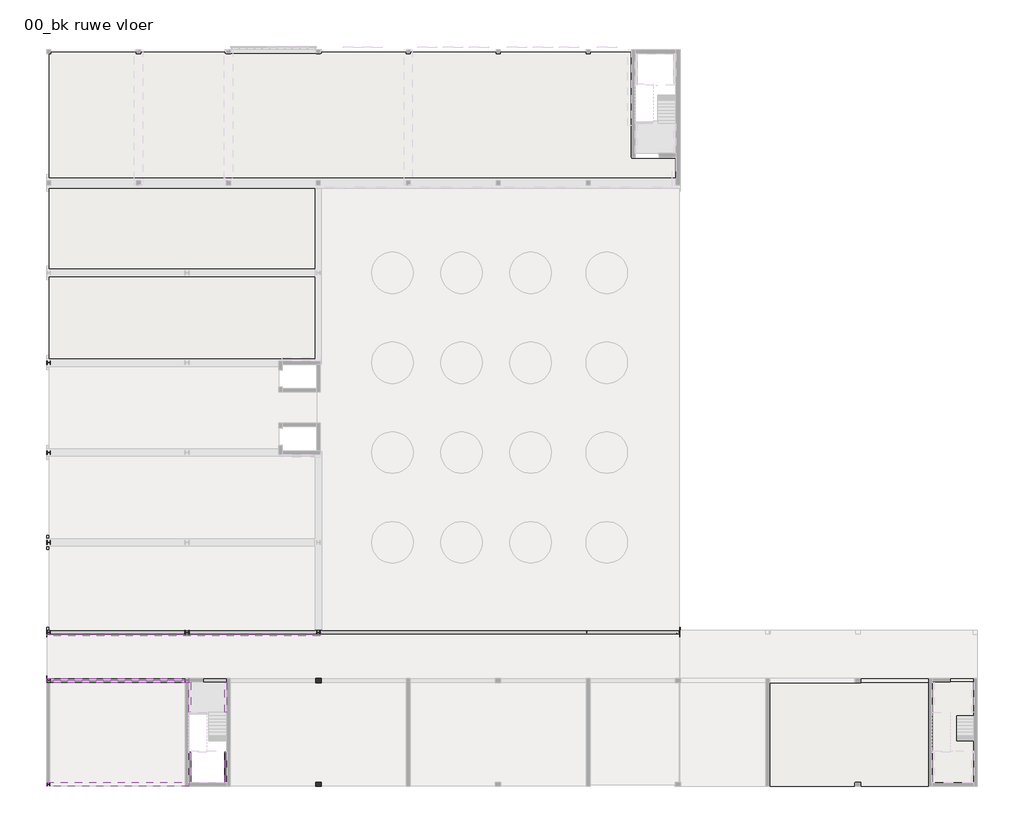
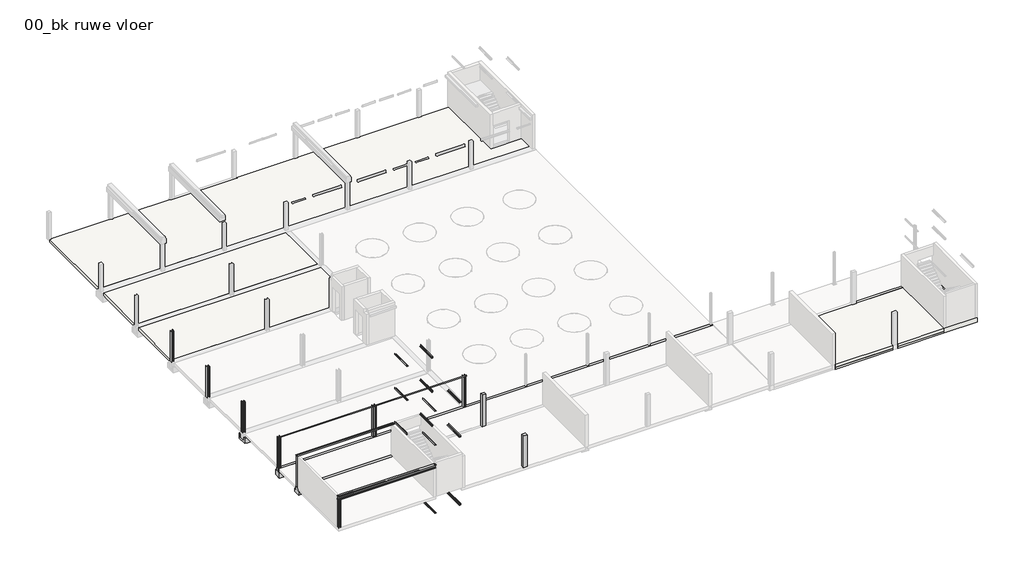
# One storey, part 4 of 6: 24 beams, 10 columns, 8 slabs.
"""IFC4 building model written with IfcOpenShell, lengths in millimetres."""

import ifcopenshell
import ifcopenshell.guid

model = None  # the IFC model being written
_history = None  # IfcOwnerHistory: only IFC2X3 demands one
_inside = {}  # id of a spatial element -> (the spatial element, [elements in it])
_under = {}  # id of a project, library or spatial element -> (it, [spatial elements below it])
_declared = {}  # id of a project -> (the project, [libraries it declares])
_typed = {}  # id of a type object -> (the type object, [elements of that type])
_made_of = {}  # id of a material, layer set ... -> (it, [elements and type objects made of it])


def new_model(schema):
    """Start an empty IFC model of exactly this schema.

    Asked for "IFC4X3", IfcOpenShell would pick the latest addendum, in which some entities
    have other attributes; the version numbers below select the first issue.
    IFC2X3 requires an IfcOwnerHistory on every rooted entity: one is made here for all.
    """
    global model, _history
    if schema == "IFC4X3":
        model = ifcopenshell.file(schema_version=(4, 3, 0, 0))
    else:
        model = ifcopenshell.file(schema=schema)
    _inside.clear()
    _under.clear()
    _declared.clear()
    _typed.clear()
    _made_of.clear()
    _history = None
    if model.schema == "IFC2X3":
        org = make("IfcOrganization", Name="unknown")
        user = make(
            "IfcPersonAndOrganization",
            ThePerson=make("IfcPerson", FamilyName="unknown"),
            TheOrganization=org,
        )
        app = make(
            "IfcApplication",
            ApplicationDeveloper=org,
            Version="unknown",
            ApplicationFullName="unknown",
            ApplicationIdentifier="unknown",
        )
        _history = make(
            "IfcOwnerHistory",
            OwningUser=user,
            OwningApplication=app,
            ChangeAction="ADDED",
            CreationDate=0,
        )
    return model


def make(cls, **values):
    """One entity of the class cls with the attributes given. An attribute that is None is left unset."""
    return model.create_entity(
        cls, **{name: value for name, value in values.items() if value is not None}
    )


def rooted(cls, **values):
    """An entity with a GlobalId (a new one), such as an element, a storey or a relation."""
    return make(cls, GlobalId=ifcopenshell.guid.new(), OwnerHistory=_history, **values)


def si_unit(unit_type, name, prefix=None):
    """IfcSIUnit, for example si_unit("LENGTHUNIT", "METRE", prefix="MILLI")."""
    return make("IfcSIUnit", UnitType=unit_type, Prefix=prefix, Name=name)


def assignment(units):
    """IfcUnitAssignment: the units of a project."""
    return None if units is None else make("IfcUnitAssignment", Units=units)


def point(xyz):
    """IfcCartesianPoint."""
    return None if xyz is None else make("IfcCartesianPoint", Coordinates=xyz)


def direction(xyz):
    """IfcDirection."""
    return None if xyz is None else make("IfcDirection", DirectionRatios=xyz)


def frame(location, z_axis=None, x_axis=None):
    """IfcAxis2Placement3D, a coordinate frame: its origin and axes. An axis left out is left unset."""
    return make(
        "IfcAxis2Placement3D",
        Location=point(location),
        Axis=direction(z_axis),
        RefDirection=direction(x_axis),
    )


def frame_2d(location, x_axis=None):
    """IfcAxis2Placement2D, a coordinate frame in the plane: its origin and x axis."""
    return make(
        "IfcAxis2Placement2D", Location=point(location), RefDirection=direction(x_axis)
    )


def origin():
    """The frame at (0, 0, 0) with its axes left unset."""
    return frame((0.0, 0.0, 0.0))


def place(relative_to, where):
    """IfcLocalPlacement: puts the frame where relative to a parent placement (None: the world)."""
    return make(
        "IfcLocalPlacement", PlacementRelTo=relative_to, RelativePlacement=where
    )


def context(
    kind, dimensions, precision=None, world=None, true_north=None, identifier=None
):
    """IfcGeometricRepresentationContext, for example the 3D "Model" context."""
    return make(
        "IfcGeometricRepresentationContext",
        ContextIdentifier=identifier,
        ContextType=kind,
        CoordinateSpaceDimension=dimensions,
        Precision=precision,
        WorldCoordinateSystem=world,
        TrueNorth=true_north,
    )


def project(units=None, contexts=None):
    """IfcProject with its units and contexts."""
    return rooted(
        "IfcProject",
        Name="project",
        RepresentationContexts=contexts,
        UnitsInContext=assignment(units),
    )


def spatial(cls, under=None, at=None, **own):
    """A site, building, storey or space (cls), placed at a placement, below another one or the project."""
    s = rooted(cls, ObjectPlacement=at, **own)
    if under is not None:
        _under.setdefault(under.id(), (under, []))[1].append(s)
    return s


def polyline(points):
    """IfcPolyline through the points."""
    return make("IfcPolyline", Points=[point(p) for p in points])


def circle_curve(where, radius):
    """IfcCircle in the frame where."""
    return make("IfcCircle", Position=where, Radius=radius)


def trimmed(basis, trim1, trim2, sense, master):
    """IfcTrimmedCurve: the piece of a basis curve between two trims."""
    return make(
        "IfcTrimmedCurve",
        BasisCurve=basis,
        Trim1=trim1,
        Trim2=trim2,
        SenseAgreement=sense,
        MasterRepresentation=master,
    )


def segment(curve, same_sense, transition):
    """IfcCompositeCurveSegment."""
    return make(
        "IfcCompositeCurveSegment",
        Transition=transition,
        SameSense=same_sense,
        ParentCurve=curve,
    )


def composite_curve(segments, self_intersect=None):
    """IfcCompositeCurve: segments joined end to end."""
    return make("IfcCompositeCurve", Segments=segments, SelfIntersect=self_intersect)


def outline(outer, holes=None, kind="AREA"):
    """IfcArbitraryClosedProfileDef: a profile drawn as a closed curve; with holes, ...WithVoids."""
    if holes is None:
        return make("IfcArbitraryClosedProfileDef", ProfileType=kind, OuterCurve=outer)
    return make(
        "IfcArbitraryProfileDefWithVoids",
        ProfileType=kind,
        OuterCurve=outer,
        InnerCurves=holes,
    )


def extrude(swept, where, along, depth):
    """IfcExtrudedAreaSolid: the profile swept, set in the frame where, extruded along a direction by depth."""
    return make(
        "IfcExtrudedAreaSolid",
        SweptArea=swept,
        Position=where,
        ExtrudedDirection=direction(along),
        Depth=depth,
    )


def faces_of(points, faces, orient=None, outer=None):
    """IfcFace entities. A face is a list of loops; a loop is a list of indices into points, from 0.

    orient and outer hold one flag for each loop. By default every Orientation is true, the
    first loop of a face is its IfcFaceOuterBound and the others are IfcFaceBound.
    """
    made = []
    for i, loops in enumerate(faces):
        bounds = []
        for j, loop in enumerate(loops):
            is_outer = j == 0 if outer is None else outer[i][j]
            bounds.append(
                make(
                    "IfcFaceOuterBound" if is_outer else "IfcFaceBound",
                    Bound=make("IfcPolyLoop", Polygon=[points[k] for k in loop]),
                    Orientation=True if orient is None else orient[i][j],
                )
            )
        made.append(make("IfcFace", Bounds=bounds))
    return made


def faceted_brep(points, faces, orient=None, outer=None, voids=None):
    """IfcFacetedBrep: a solid bounded by flat faces; with voids (closed shells), ...WithVoids."""
    shared = [point(p) for p in points]
    hull = make("IfcClosedShell", CfsFaces=faces_of(shared, faces, orient, outer))
    if voids is None:
        return make("IfcFacetedBrep", Outer=hull)
    return make(
        "IfcFacetedBrepWithVoids",
        Outer=hull,
        Voids=[
            make(cls, CfsFaces=faces_of(shared, fs, o, b)) for cls, fs, o, b in voids
        ],
    )


def shape(context_of_items, identifier, shape_type, items):
    """IfcShapeRepresentation: the items that make up one representation, for example the "Body"."""
    return make(
        "IfcShapeRepresentation",
        ContextOfItems=context_of_items,
        RepresentationIdentifier=identifier,
        RepresentationType=shape_type,
        Items=items,
    )


def source(mapping_origin, context_of_items, identifier, shape_type, items):
    """IfcRepresentationMap: a shape defined once, which mapped items show again and again."""
    return make(
        "IfcRepresentationMap",
        MappingOrigin=mapping_origin,
        MappedRepresentation=shape(context_of_items, identifier, shape_type, items),
    )


def transform(
    local_origin,
    x_axis=None,
    y_axis=None,
    z_axis=None,
    scale=None,
    scale2=None,
    scale3=None,
    uniform=True,
):
    """IfcCartesianTransformationOperator3D, or its non-uniform kind. x_axis, y_axis, z_axis: its Axis1, 2, 3."""
    if uniform:
        return make(
            "IfcCartesianTransformationOperator3D",
            Axis1=direction(x_axis),
            Axis2=direction(y_axis),
            LocalOrigin=point(local_origin),
            Scale=scale,
            Axis3=direction(z_axis),
        )
    return make(
        "IfcCartesianTransformationOperator3DnonUniform",
        Axis1=direction(x_axis),
        Axis2=direction(y_axis),
        LocalOrigin=point(local_origin),
        Scale=scale,
        Axis3=direction(z_axis),
        Scale2=scale2,
        Scale3=scale3,
    )


def mapped(mapping_source, mapping_target):
    """IfcMappedItem: shows the shape of a source again, moved by a transform."""
    return make(
        "IfcMappedItem", MappingSource=mapping_source, MappingTarget=mapping_target
    )


def made_of(thing, what):
    """Note that an element or type object is made of a material, layer set ...; save() writes the relation."""
    if what is not None:
        _made_of.setdefault(what.id(), (what, []))[1].append(thing)
    return thing


def element(
    cls,
    number,
    at=None,
    inside=None,
    cuts=None,
    type_object=None,
    material=None,
    context=None,
    identifier="Body",
    shape_type=None,
    held_by="IfcProductDefinitionShape",
    body=None,
    shapes=None,
    **own,
):
    """One element of the class cls, such as IfcWall. Its Tag is "e" and its number.

    at: its placement. inside: the storey or other place that contains it. cuts: it is an
    opening in that element (IfcRelVoidsElement). A single representation is given by context,
    identifier, shape_type and body (its items); several are given by shapes. held_by: the class
    of the entity that holds the representations. save() writes the other relations.
    """
    e = rooted(cls, Tag="e%d" % number, ObjectPlacement=at, **own)
    if body is not None:
        shapes = [shape(context, identifier, shape_type, body)]
    if shapes is not None:
        e.Representation = make(held_by, Representations=shapes)
    if inside is not None:
        _inside.setdefault(inside.id(), (inside, []))[1].append(e)
    if cuts is not None:
        rooted(
            "IfcRelVoidsElement", RelatingBuildingElement=cuts, RelatedOpeningElement=e
        )
    if type_object is not None:
        _typed.setdefault(type_object.id(), (type_object, []))[1].append(e)
    return made_of(e, material)


def aggregate(whole, parts):
    """IfcRelAggregates: a whole, such as a stair, and the parts it consists of."""
    return rooted("IfcRelAggregates", RelatingObject=whole, RelatedObjects=parts)


def save(model, path):
    """Write the relations noted so far, then the file.

    IfcRelAggregates (storeys below a building ...), IfcRelContainedInSpatialStructure (elements
    in a storey), IfcRelDefinesByType, IfcRelAssociatesMaterial and IfcRelDeclares: one each for
    every whole, place, type object, material and project.
    """
    for whole, parts in _under.values():
        aggregate(whole, parts)
    for where, things in _inside.values():
        rooted(
            "IfcRelContainedInSpatialStructure",
            RelatedElements=things,
            RelatingStructure=where,
        )
    for kind, things in _typed.values():
        rooted("IfcRelDefinesByType", RelatedObjects=things, RelatingType=kind)
    for what, things in _made_of.values():
        rooted("IfcRelAssociatesMaterial", RelatedObjects=things, RelatingMaterial=what)
    for by, libraries in _declared.values():
        rooted("IfcRelDeclares", RelatingContext=by, RelatedDefinitions=libraries)
    model.write(path)


def beam_86464b0d(model_context):
    return source(origin(), model_context, "Body", "SweptSolid", [
        extrude(outline(composite_curve([segment(polyline([(-42.5, -42.5), (-42.5, 107.5), (-35.5, 107.5)]), True, "CONTINUOUS"), segment(trimmed(circle_curve(frame_2d((-35.5, 99.5)), 8.0), [point((-35.5, 107.5))], [point((-27.5, 99.5))], False, "CARTESIAN"), True, "CONTINUOUS"), segment(polyline([(-27.5, 99.5), (-27.5, -11.5)]), True, "CONTINUOUS"), segment(trimmed(circle_curve(frame_2d((-11.5, -11.5)), 16.0), [point((-27.5, -11.5))], [point((-11.5, -27.5))], True, "CARTESIAN"), True, "CONTINUOUS"), segment(polyline([(-11.5, -27.5), (99.5, -27.5)]), True, "CONTINUOUS"), segment(trimmed(circle_curve(frame_2d((99.5, -35.5)), 8.0), [point((99.5, -27.5))], [point((107.5, -35.5))], False, "CARTESIAN"), True, "CONTINUOUS"), segment(polyline([(107.5, -35.5), (107.5, -42.5), (-42.5, -42.5)]), True, "CONTINUOUS")], self_intersect=False)), frame((-1095.0, 0.0, 0.0), z_axis=(1.0, 0.0, 0.0), x_axis=(0.0, 1.0, 0.0)), (0.0, 0.0, 1.0), 2190.0),
    ])


def beam_a9a0024c(model_context):
    return source(origin(), model_context, "Body", "SweptSolid", [
        extrude(outline(composite_curve([segment(polyline([(42.5, -42.5), (-107.5, -42.5), (-107.5, -35.5)]), True, "CONTINUOUS"), segment(trimmed(circle_curve(frame_2d((-99.5, -35.5)), 8.0), [point((-107.5, -35.5))], [point((-99.5, -27.5))], False, "CARTESIAN"), True, "CONTINUOUS"), segment(polyline([(-99.5, -27.5), (11.5, -27.5)]), True, "CONTINUOUS"), segment(trimmed(circle_curve(frame_2d((11.5, -11.5)), 16.0), [point((11.5, -27.5))], [point((27.5, -11.5))], True, "CARTESIAN"), True, "CONTINUOUS"), segment(polyline([(27.5, -11.5), (27.5, 99.5)]), True, "CONTINUOUS"), segment(trimmed(circle_curve(frame_2d((35.5, 99.5)), 8.0), [point((27.5, 99.5))], [point((35.5, 107.5))], False, "CARTESIAN"), True, "CONTINUOUS"), segment(polyline([(35.5, 107.5), (42.5, 107.5), (42.5, -42.5)]), True, "CONTINUOUS")], self_intersect=False)), frame((-1095.0, 0.0, 0.0), z_axis=(1.0, 0.0, 0.0), x_axis=(0.0, 1.0, 0.0)), (0.0, 0.0, 1.0), 2190.0),
    ])


model = new_model("IFC4")

# Units and contexts
model_context = context("Model", 3, world=origin())
ifc_project = project(units=[si_unit("LENGTHUNIT", "METRE", prefix="MILLI")], contexts=[model_context])

# Site, building, storey
site = spatial("IfcSite", under=ifc_project)
building = spatial("IfcBuilding", under=site)
storey = spatial("IfcBuildingStorey", under=building, Name="00_bk ruwe vloer", Elevation=-70.0)

# Beams
placement = place(None, origin())
element("IfcBeam", 1, ObjectType="NLRS_28_SF_LIB_balk dubbele sponning beton prefab-CWV-MMBC-SRP_gen_rsf : balk beton prefab_gen__bxh 700x900 met inkassing bxh 200x320", at=placement, inside=storey, context=model_context, shape_type="Brep", body=[
    faceted_brep([(52150.0, 11150.0, -70.0), (52150.0, 10850.0, -70.0), (52150.0, 10850.0, -390.0), (52150.0, 10650.0, -390.0), (52150.0, 10650.0, -970.0), (52150.0, 11350.0, -970.0), (52150.0, 11350.0, -390.0), (52150.0, 11150.0, -390.0), (6350.0, 11150.0, -70.0), (6350.0, 11150.0, -390.0), (6350.0, 11350.0, -390.0), (6350.0, 11350.0, -970.0), (6350.0, 10650.0, -970.0), (6350.0, 10650.0, -390.0), (6350.0, 10850.0, -390.0), (6350.0, 10850.0, -70.0), (52090.0, 11150.0, -70.0), (26300.0, 11150.0, -70.0), (25750.0, 11150.0, -70.0), (6550.0, 11150.0, -70.0), (6410.0, 10850.0, -70.0), (52090.0, 10850.0, -70.0), (6410.0, 10850.0, -390.0), (52090.0, 10850.0, -390.0), (6410.0, 10650.0, -390.0), (6625.0, 10650.0, -390.0), (6650.0, 10650.0, -390.0), (51850.0, 10650.0, -390.0), (51875.0, 10650.0, -390.0), (52090.0, 10650.0, -390.0), (6650.0, 10650.0, -970.0), (51850.0, 10650.0, -970.0), (6650.0, 11350.0, -970.0), (25500.0, 11350.0, -970.0), (26500.0, 11350.0, -970.0), (51850.0, 11350.0, -970.0), (6550.0, 11350.0, -390.0), (6650.0, 11350.0, -390.0), (25500.0, 11350.0, -390.0), (25750.0, 11350.0, -390.0), (26300.0, 11350.0, -390.0), (26425.0, 11350.0, -390.0), (26500.0, 11350.0, -390.0), (51850.0, 11350.0, -390.0), (51875.0, 11350.0, -390.0), (52090.0, 11350.0, -390.0), (6550.0, 11150.0, -390.0), (25750.0, 11150.0, -390.0), (26300.0, 11150.0, -390.0), (52090.0, 11150.0, -390.0)], [[[0, 1, 2, 3, 4, 5, 6, 7]], [[8, 9, 10, 11, 12, 13, 14, 15]], [[1, 0, 16, 17, 18, 19, 8, 15, 20, 21]], [[2, 1, 21, 20, 15, 14, 22, 23]], [[3, 2, 23, 22, 14, 13, 24, 25, 26, 27, 28, 29]], [[4, 3, 29, 28, 27, 26, 25, 24, 13, 12, 30, 31]], [[5, 4, 31, 30, 12, 11, 32, 33, 34, 35]], [[6, 5, 35, 34, 33, 32, 11, 10, 36, 37, 38, 39, 40, 41, 42, 43, 44, 45]], [[7, 6, 45, 44, 43, 42, 41, 40, 39, 38, 37, 36, 10, 9, 46, 47, 48, 49]], [[0, 7, 49, 48, 47, 46, 9, 8, 19, 18, 17, 16]]]),
])
element("IfcBeam", 2, ObjectType="NLRS_28_SF_LIB_balkbodem beton prefab-CWV-MMBC-SRP_gen_rsf : balkbodem beton prefab_gen__bxhxdk 1000x580x200", at=placement, inside=storey, context=model_context, shape_type="Brep", body=[
    faceted_brep([(25550.0, 17000.0, -390.0), (25550.0, 17000.0, -970.0), (25550.0, 18000.0, -970.0), (25550.0, 18000.0, -390.0), (25550.0, 17800.0, -390.0), (25550.0, 17800.0, -770.0), (25550.0, 17200.0, -770.0), (25550.0, 17200.0, -390.0), (6350.0, 17000.0, -390.0), (6350.0, 17200.0, -390.0), (6350.0, 17200.0, -770.0), (6350.0, 17800.0, -770.0), (6350.0, 17800.0, -390.0), (6350.0, 18000.0, -390.0), (6350.0, 18000.0, -970.0), (6350.0, 17000.0, -970.0), (25500.0, 17000.0, -390.0), (6650.0, 17000.0, -390.0), (6550.0, 17000.0, -390.0), (6650.0, 17000.0, -970.0), (25500.0, 17000.0, -970.0), (6650.0, 18000.0, -970.0), (25500.0, 18000.0, -970.0), (6550.0, 18000.0, -390.0), (6650.0, 18000.0, -390.0), (25500.0, 18000.0, -390.0), (6550.0, 17800.0, -390.0), (25500.0, 17800.0, -390.0), (25500.0, 17800.0, -770.0), (25500.0, 17200.0, -770.0), (6550.0, 17200.0, -390.0), (25500.0, 17200.0, -390.0)], [[[0, 1, 2, 3, 4, 5, 6, 7]], [[8, 9, 10, 11, 12, 13, 14, 15]], [[1, 0, 16, 17, 18, 8, 15, 19, 20]], [[2, 1, 20, 19, 15, 14, 21, 22]], [[3, 2, 22, 21, 14, 13, 23, 24, 25]], [[4, 3, 25, 24, 23, 13, 12, 26, 27]], [[5, 4, 27, 26, 12, 11, 28]], [[6, 5, 28, 11, 10, 29]], [[7, 6, 29, 10, 9, 30, 31]], [[0, 7, 31, 30, 9, 8, 18, 17, 16]]]),
])
element("IfcBeam", 3, ObjectType="NLRS_28_SF_LIB_balk dubbele sponning beton prefab-CWV-MMBC-SRP_gen_rsf : balk beton prefab_gen__bxh 700x700 met inkassing bxh 200x320", at=placement, inside=storey, context=model_context, shape_type="Brep", body=[
    faceted_brep([(6350.0, 7650.0, -70.0), (6350.0, 7650.0, -390.0), (6350.0, 7850.0, -390.0), (6350.0, 7850.0, -770.0), (6350.0, 7150.0, -770.0), (6350.0, 7150.0, -390.0), (6350.0, 7350.0, -390.0), (6350.0, 7350.0, -70.0), (6410.0, 7350.0, -70.0), (16625.0, 7350.0, -70.0), (16625.0, 7400.0, -70.0), (16625.0, 7650.0, -70.0), (16375.0, 7650.0, -70.0), (6410.0, 7650.0, -70.0), (6410.0, 7350.0, -390.0), (16375.0, 7350.0, -390.0), (16625.0, 7350.0, -390.0), (6410.0, 7150.0, -390.0), (6625.0, 7150.0, -390.0), (6650.0, 7150.0, -390.0), (16375.0, 7150.0, -390.0), (6650.0, 7150.0, -770.0), (16375.0, 7150.0, -770.0), (6650.0, 7850.0, -770.0), (16625.0, 7850.0, -770.0), (16625.0, 7650.0, -770.0), (16375.0, 7650.0, -770.0), (6410.0, 7850.0, -390.0), (6625.0, 7850.0, -390.0), (6650.0, 7850.0, -390.0), (16625.0, 7850.0, -390.0), (6410.0, 7650.0, -390.0), (16375.0, 7650.0, -390.0), (16625.0, 7650.0, -390.0), (16625.0, 7825.0, -390.0), (16375.0, 7650.0, -390.0)], [[[0, 1, 2, 3, 4, 5, 6, 7]], [[0, 7, 8, 9, 10, 11, 12, 13]], [[7, 6, 14, 15, 16, 9, 8]], [[6, 5, 17, 18, 19, 20, 15, 14]], [[5, 4, 21, 22, 20, 19, 18, 17]], [[4, 3, 23, 24, 25, 26, 22, 21]], [[3, 2, 27, 28, 29, 30, 24, 23]], [[2, 1, 31, 32, 33, 34, 30, 29, 28, 27]], [[1, 0, 13, 12, 11, 33, 32, 31]], [[11, 10, 9, 16, 33]], [[35, 15, 20, 22, 26]], [[35, 33, 16, 15]], [[33, 35, 26, 25]], [[24, 30, 34, 33, 25]]]),
])
element("IfcBeam", 4, ObjectType="NLRS_28_SF_LIB_balk dubbele sponning beton prefab-CWV-MMBC-SRP_gen_rsf : balk beton prefab_gen__bxh 700x700 met inkassing bxh 200x320", at=placement, inside=storey, context=model_context, shape_type="Brep", body=[
    faceted_brep([(16625.0, 7650.0, -70.0), (16625.0, 7650.0, -390.0), (16625.0, 7825.0, -390.0), (16625.0, 7850.0, -390.0), (16625.0, 7850.0, -770.0), (16625.0, 7650.0, -770.0), (16625.0, 7400.0, -770.0), (16625.0, 7400.0, -70.0), (17675.0, 7400.0, -70.0), (19375.0, 7400.0, -70.0), (19375.0, 7650.0, -70.0), (17675.0, 7650.0, -70.0), (19375.0, 7850.0, -770.0), (19375.0, 7650.0, -770.0), (19375.0, 7400.0, -770.0), (19375.0, 7850.0, -390.0), (19375.0, 7650.0, -390.0), (19375.0, 7825.0, -390.0)], [[[0, 1, 2, 3, 4, 5, 6, 7]], [[0, 7, 8, 9, 10, 11]], [[6, 5, 4, 12, 13, 14]], [[4, 3, 15, 12]], [[15, 3, 2, 1, 16, 17]], [[1, 0, 11, 10, 16]], [[7, 6, 14, 9, 8]], [[10, 9, 14, 13, 12, 15, 17, 16]]]),
])
element("IfcBeam", 5, ObjectType="NLRS_28_SF_LIB_stalen ligger HEB-AV-CWV-MMBS-SRP_gen_rsf : stalen ligger_gen__HEB 360", at=placement, inside=storey, context=model_context, shape_type="SweptSolid", body=[
    extrude(outline(composite_curve([segment(polyline([(150.0, 3447.5), (33.25, 3447.5)]), True, "CONTINUOUS"), segment(trimmed(circle_curve(frame_2d((33.25, 3420.5)), 27.0), [point((33.25, 3447.5))], [point((6.25, 3420.5))], True, "CARTESIAN"), True, "CONTINUOUS"), segment(polyline([(6.25, 3420.5), (6.25, 3159.5)]), True, "CONTINUOUS"), segment(trimmed(circle_curve(frame_2d((33.25, 3159.5)), 27.0), [point((6.25, 3159.5))], [point((33.25, 3132.5))], True, "CARTESIAN"), True, "CONTINUOUS"), segment(polyline([(33.25, 3132.5), (150.0, 3132.5), (150.0, 3110.0), (-150.0, 3110.0), (-150.0, 3132.5), (-33.25, 3132.5)]), True, "CONTINUOUS"), segment(trimmed(circle_curve(frame_2d((-33.25, 3159.5)), 27.0), [point((-33.25, 3132.5))], [point((-6.25, 3159.5))], True, "CARTESIAN"), True, "CONTINUOUS"), segment(polyline([(-6.25, 3159.5), (-6.25, 3420.5)]), True, "CONTINUOUS"), segment(trimmed(circle_curve(frame_2d((-33.25, 3420.5)), 27.0), [point((-6.25, 3420.5))], [point((-33.25, 3447.5))], True, "CARTESIAN"), True, "CONTINUOUS"), segment(polyline([(-33.25, 3447.5), (-150.0, 3447.5), (-150.0, 3470.0), (150.0, 3470.0), (150.0, 3447.5)]), True, "CONTINUOUS")], self_intersect=False)), frame((6350.0, 0.0, 0.0), z_axis=(1.0, 0.0, 0.0), x_axis=(0.0, 1.0, 0.0)), (0.0, 0.0, 1.0), 10275.0),
])
element("IfcBeam", 6, ObjectType="NLRS_28_SF_LIB_stalen ligger stripstaal-AV-MMBS-SRP_gen_rsf : stalen ligger stripstaal RECT_gen__140x15", at=placement, inside=storey, context=model_context, shape_type="SweptSolid", body=[
    extrude(outline(polyline([(16625.0, 7493.0), (16625.0, 7353.0), (6350.0, 7353.0), (6350.0, 7493.0), (16625.0, 7493.0)])), frame((0.0, 0.0, 3455.0), z_axis=(0.0, 0.0, 1.0), x_axis=(1.0, 0.0, 0.0)), (0.0, 0.0, 1.0), 15.0),
    extrude(outline(polyline([(16625.0, 7493.0), (16625.0, 7353.0), (6350.0, 7353.0), (6350.0, 7493.0), (16625.0, 7493.0)])), frame((0.0, 0.0, 3455.0), z_axis=(0.0, 0.0, 1.0), x_axis=(1.0, 0.0, 0.0)), (0.0, 0.0, 1.0), 15.0),
])
element("IfcBeam", 7, ObjectType="NLRS_28_SF_LIB_stalen ligger stripstaal-AV-MMBS-SRP_gen_rsf : stalen ligger stripstaal RECT_gen__140x15", at=placement, inside=storey, context=model_context, shape_type="SweptSolid", body=[
    extrude(outline(polyline([(16625.0, 7507.0), (6350.0, 7507.0), (6350.0, 7647.0), (16625.0, 7647.0), (16625.0, 7507.0)])), frame((0.0, 0.0, 3455.0), z_axis=(0.0, 0.0, 1.0), x_axis=(1.0, 0.0, 0.0)), (0.0, 0.0, 1.0), 15.0),
    extrude(outline(polyline([(16625.0, 7507.0), (6350.0, 7507.0), (6350.0, 7647.0), (16625.0, 7647.0), (16625.0, 7507.0)])), frame((0.0, 0.0, 3455.0), z_axis=(0.0, 0.0, 1.0), x_axis=(1.0, 0.0, 0.0)), (0.0, 0.0, 1.0), 15.0),
])
element("IfcBeam", 8, ObjectType="NLRS_28_SF_LIB_stalen ligger stripstaal-AV-MMBS-SRP_gen_rsf : stalen ligger stripstaal RECT_gen__120x15", at=placement, inside=storey, context=model_context, shape_type="SweptSolid", body=[
    extrude(outline(polyline([(26125.0, 10856.5), (26125.0, 10736.5), (6350.0, 10736.5), (6350.0, 10856.5), (26125.0, 10856.5)])), frame((0.0, 0.0, 3455.0), z_axis=(0.0, 0.0, 1.0), x_axis=(1.0, 0.0, 0.0)), (0.0, 0.0, 1.0), 15.0),
    extrude(outline(polyline([(26125.0, 10856.5), (26125.0, 10736.5), (6350.0, 10736.5), (6350.0, 10856.5), (26125.0, 10856.5)])), frame((0.0, 0.0, 3455.0), z_axis=(0.0, 0.0, 1.0), x_axis=(1.0, 0.0, 0.0)), (0.0, 0.0, 1.0), 15.0),
])
beam_shape = beam_86464b0d(model_context)
element("IfcBeam", 9, ObjectType="NLRS_28_SF_LIB_stalen ligger hoekprofiel gelijkzijdig-AV-MMBS-SRP_gen_rsf : stalen ligger gelijkzijdig hoekprofiel LEQU_gen__150x150x15", at=placement, inside=storey, context=model_context, shape_type="MappedRepresentation", body=[
    mapped(beam_shape, transform((19332.5, 1205.0, 1722.5), x_axis=(0.0, 1.0, 0.0), y_axis=(-1.0, 0.0, 0.0), z_axis=(0.0, 0.0, 1.0))),
])
element("IfcBeam", 10, ObjectType="NLRS_28_SF_LIB_stalen ligger hoekprofiel gelijkzijdig-AV-MMBS-SRP_gen_rsf : stalen ligger gelijkzijdig hoekprofiel LEQU_gen__150x150x15", at=placement, inside=storey, context=model_context, shape_type="MappedRepresentation", body=[
    mapped(beam_shape, transform((19332.5, 1205.0, -2077.5), x_axis=(0.0, 1.0, 0.0), y_axis=(-1.0, 0.0, 0.0), z_axis=(0.0, 0.0, 1.0))),
])
element("IfcBeam", 11, ObjectType="NLRS_28_SF_LIB_stalen ligger hoekprofiel gelijkzijdig-AV-MMBS-SRP_gen_rsf : stalen ligger gelijkzijdig hoekprofiel LEQU_gen__150x150x15", at=placement, inside=storey, context=model_context, shape_type="MappedRepresentation", body=[
    mapped(beam_shape, transform((19332.5, 1205.0, 5522.5), x_axis=(0.0, 1.0, 0.0), y_axis=(-1.0, 0.0, 0.0), z_axis=(0.0, 0.0, 1.0))),
])
element("IfcBeam", 12, ObjectType="NLRS_28_SF_LIB_stalen ligger hoekprofiel gelijkzijdig-AV-MMBS-SRP_gen_rsf : stalen ligger gelijkzijdig hoekprofiel LEQU_gen__150x150x15", at=placement, inside=storey, context=model_context, shape_type="MappedRepresentation", body=[
    mapped(beam_shape, transform((19332.5, 1205.0, 9322.5), x_axis=(0.0, 1.0, 0.0), y_axis=(-1.0, 0.0, 0.0), z_axis=(0.0, 0.0, 1.0))),
])
element("IfcBeam", 13, ObjectType="NLRS_28_SF_LIB_stalen ligger hoekprofiel gelijkzijdig-AV-MMBS-SRP_gen_rsf : stalen ligger gelijkzijdig hoekprofiel LEQU_gen__150x150x15", at=placement, inside=storey, context=model_context, shape_type="MappedRepresentation", body=[
    mapped(beam_shape, transform((19332.5, 6295.0, -177.5), x_axis=(0.0, 1.0, 0.0), y_axis=(-1.0, 0.0, 0.0), z_axis=(0.0, 0.0, 1.0))),
])
element("IfcBeam", 14, ObjectType="NLRS_28_SF_LIB_stalen ligger hoekprofiel gelijkzijdig-AV-MMBS-SRP_gen_rsf : stalen ligger gelijkzijdig hoekprofiel LEQU_gen__150x150x15", at=placement, inside=storey, context=model_context, shape_type="MappedRepresentation", body=[
    mapped(beam_shape, transform((19332.5, 6295.0, 3622.5), x_axis=(0.0, 1.0, 0.0), y_axis=(-1.0, 0.0, 0.0), z_axis=(0.0, 0.0, 1.0))),
])
element("IfcBeam", 15, ObjectType="NLRS_28_SF_LIB_stalen ligger hoekprofiel gelijkzijdig-AV-MMBS-SRP_gen_rsf : stalen ligger gelijkzijdig hoekprofiel LEQU_gen__150x150x15", at=placement, inside=storey, context=model_context, shape_type="MappedRepresentation", body=[
    mapped(beam_shape, transform((19332.5, 6295.0, 7422.5), x_axis=(0.0, 1.0, 0.0), y_axis=(-1.0, 0.0, 0.0), z_axis=(0.0, 0.0, 1.0))),
])
element("IfcBeam", 16, ObjectType="NLRS_28_SF_LIB_stalen ligger hoekprofiel gelijkzijdig-AV-MMBS-SRP_gen_rsf : stalen ligger gelijkzijdig hoekprofiel LEQU_gen__150x150x15", at=placement, inside=storey, context=model_context, shape_type="MappedRepresentation", body=[
    mapped(beam_shape, transform((19332.5, 6295.0, 11222.5), x_axis=(0.0, 1.0, 0.0), y_axis=(-1.0, 0.0, 0.0), z_axis=(0.0, 0.0, 1.0))),
])
beam_2_shape = beam_a9a0024c(model_context)
element("IfcBeam", 17, ObjectType="NLRS_28_SF_LIB_stalen ligger hoekprofiel gelijkzijdig-AV-MMBS-SRP_gen_rsf : stalen ligger gelijkzijdig hoekprofiel LEQU_gen__150x150x15", at=placement, inside=storey, context=model_context, shape_type="MappedRepresentation", body=[
    mapped(beam_2_shape, transform((16667.5, 1205.0, 1722.5), x_axis=(0.0, 1.0, 0.0), y_axis=(-1.0, 0.0, 0.0), z_axis=(0.0, 0.0, 1.0))),
])
element("IfcBeam", 18, ObjectType="NLRS_28_SF_LIB_stalen ligger hoekprofiel gelijkzijdig-AV-MMBS-SRP_gen_rsf : stalen ligger gelijkzijdig hoekprofiel LEQU_gen__150x150x15", at=placement, inside=storey, context=model_context, shape_type="MappedRepresentation", body=[
    mapped(beam_2_shape, transform((16667.5, 1205.0, -2077.5), x_axis=(0.0, 1.0, 0.0), y_axis=(-1.0, 0.0, 0.0), z_axis=(0.0, 0.0, 1.0))),
])
element("IfcBeam", 19, ObjectType="NLRS_28_SF_LIB_stalen ligger hoekprofiel gelijkzijdig-AV-MMBS-SRP_gen_rsf : stalen ligger gelijkzijdig hoekprofiel LEQU_gen__150x150x15", at=placement, inside=storey, context=model_context, shape_type="MappedRepresentation", body=[
    mapped(beam_2_shape, transform((16667.5, 1205.0, 5522.5), x_axis=(0.0, 1.0, 0.0), y_axis=(-1.0, 0.0, 0.0), z_axis=(0.0, 0.0, 1.0))),
])
element("IfcBeam", 20, ObjectType="NLRS_28_SF_LIB_stalen ligger hoekprofiel gelijkzijdig-AV-MMBS-SRP_gen_rsf : stalen ligger gelijkzijdig hoekprofiel LEQU_gen__150x150x15", at=placement, inside=storey, context=model_context, shape_type="MappedRepresentation", body=[
    mapped(beam_2_shape, transform((16667.5, 1205.0, 9322.5), x_axis=(0.0, 1.0, 0.0), y_axis=(-1.0, 0.0, 0.0), z_axis=(0.0, 0.0, 1.0))),
])
element("IfcBeam", 21, ObjectType="NLRS_28_SF_LIB_stalen ligger hoekprofiel gelijkzijdig-AV-MMBS-SRP_gen_rsf : stalen ligger gelijkzijdig hoekprofiel LEQU_gen__150x150x15", at=placement, inside=storey, context=model_context, shape_type="MappedRepresentation", body=[
    mapped(beam_2_shape, transform((16667.5, 6295.0, -177.5), x_axis=(0.0, 1.0, 0.0), y_axis=(-1.0, 0.0, 0.0), z_axis=(0.0, 0.0, 1.0))),
])
element("IfcBeam", 22, ObjectType="NLRS_28_SF_LIB_stalen ligger hoekprofiel gelijkzijdig-AV-MMBS-SRP_gen_rsf : stalen ligger gelijkzijdig hoekprofiel LEQU_gen__150x150x15", at=placement, inside=storey, context=model_context, shape_type="MappedRepresentation", body=[
    mapped(beam_2_shape, transform((16667.5, 6295.0, 3622.5), x_axis=(0.0, 1.0, 0.0), y_axis=(-1.0, 0.0, 0.0), z_axis=(0.0, 0.0, 1.0))),
])
element("IfcBeam", 23, ObjectType="NLRS_28_SF_LIB_stalen ligger hoekprofiel gelijkzijdig-AV-MMBS-SRP_gen_rsf : stalen ligger gelijkzijdig hoekprofiel LEQU_gen__150x150x15", at=placement, inside=storey, context=model_context, shape_type="MappedRepresentation", body=[
    mapped(beam_2_shape, transform((16667.5, 6295.0, 7422.5), x_axis=(0.0, 1.0, 0.0), y_axis=(-1.0, 0.0, 0.0), z_axis=(0.0, 0.0, 1.0))),
])
element("IfcBeam", 24, ObjectType="NLRS_28_SF_LIB_stalen ligger hoekprofiel gelijkzijdig-AV-MMBS-SRP_gen_rsf : stalen ligger gelijkzijdig hoekprofiel LEQU_gen__150x150x15", at=placement, inside=storey, context=model_context, shape_type="MappedRepresentation", body=[
    mapped(beam_2_shape, transform((16667.5, 6295.0, 11222.5), x_axis=(0.0, 1.0, 0.0), y_axis=(-1.0, 0.0, 0.0), z_axis=(0.0, 0.0, 1.0))),
])

# Columns
element("IfcColumn", 25, ObjectType="NLRS_28_SCO_TLB_stalen kolom HEA-BCPG-MMBS-SRP_gen_rsf : stalen kolom_gen__HEA 260", at=placement, inside=storey, context=model_context, shape_type="SweptSolid", body=[
    extrude(outline(composite_curve([segment(polyline([(6375.0, 11130.0), (6387.5, 11130.0), (6387.5, 11027.75)]), True, "CONTINUOUS"), segment(trimmed(circle_curve(frame_2d((6411.5, 11027.75)), 24.0), [point((6387.5, 11027.75))], [point((6411.5, 11003.75))], True, "CARTESIAN"), True, "CONTINUOUS"), segment(polyline([(6411.5, 11003.75), (6588.5, 11003.75)]), True, "CONTINUOUS"), segment(trimmed(circle_curve(frame_2d((6588.5, 11027.75)), 24.0), [point((6588.5, 11003.75))], [point((6612.5, 11027.75))], True, "CARTESIAN"), True, "CONTINUOUS"), segment(polyline([(6612.5, 11027.75), (6612.5, 11130.0), (6625.0, 11130.0), (6625.0, 10870.0), (6612.5, 10870.0), (6612.5, 10972.25)]), True, "CONTINUOUS"), segment(trimmed(circle_curve(frame_2d((6588.5, 10972.25)), 24.0), [point((6612.5, 10972.25))], [point((6588.5, 10996.25))], True, "CARTESIAN"), True, "CONTINUOUS"), segment(polyline([(6588.5, 10996.25), (6411.5, 10996.25)]), True, "CONTINUOUS"), segment(trimmed(circle_curve(frame_2d((6411.5, 10972.25)), 24.0), [point((6411.5, 10996.25))], [point((6387.5, 10972.25))], True, "CARTESIAN"), True, "CONTINUOUS"), segment(polyline([(6387.5, 10972.25), (6387.5, 10870.0), (6375.0, 10870.0), (6375.0, 11130.0)]), True, "CONTINUOUS")], self_intersect=False)), frame((0.0, 0.0, -40.0), z_axis=(0.0, 0.0, 1.0), x_axis=(1.0, 0.0, 0.0)), (0.0, 0.0, 1.0), 3420.0),
])
element("IfcColumn", 26, ObjectType="NLRS_28_SCO_TLB_stalen kolom HEA-BCPG-MMBS-SRP_gen_rsf : stalen kolom_gen__HEA 260", at=placement, inside=storey, context=model_context, shape_type="SweptSolid", body=[
    extrude(outline(composite_curve([segment(polyline([(6375.0, 17630.0), (6387.5, 17630.0), (6387.5, 17527.75)]), True, "CONTINUOUS"), segment(trimmed(circle_curve(frame_2d((6411.5, 17527.75)), 24.0), [point((6387.5, 17527.75))], [point((6411.5, 17503.75))], True, "CARTESIAN"), True, "CONTINUOUS"), segment(polyline([(6411.5, 17503.75), (6588.5, 17503.75)]), True, "CONTINUOUS"), segment(trimmed(circle_curve(frame_2d((6588.5, 17527.75)), 24.0), [point((6588.5, 17503.75))], [point((6612.5, 17527.75))], True, "CARTESIAN"), True, "CONTINUOUS"), segment(polyline([(6612.5, 17527.75), (6612.5, 17630.0), (6625.0, 17630.0), (6625.0, 17370.0), (6612.5, 17370.0), (6612.5, 17472.25)]), True, "CONTINUOUS"), segment(trimmed(circle_curve(frame_2d((6588.5, 17472.25)), 24.0), [point((6612.5, 17472.25))], [point((6588.5, 17496.25))], True, "CARTESIAN"), True, "CONTINUOUS"), segment(polyline([(6588.5, 17496.25), (6411.5, 17496.25)]), True, "CONTINUOUS"), segment(trimmed(circle_curve(frame_2d((6411.5, 17472.25)), 24.0), [point((6411.5, 17496.25))], [point((6387.5, 17472.25))], True, "CARTESIAN"), True, "CONTINUOUS"), segment(polyline([(6387.5, 17472.25), (6387.5, 17370.0), (6375.0, 17370.0), (6375.0, 17630.0)]), True, "CONTINUOUS")], self_intersect=False)), frame((0.0, 0.0, -40.0), z_axis=(0.0, 0.0, 1.0), x_axis=(1.0, 0.0, 0.0)), (0.0, 0.0, 1.0), 3420.0),
])
element("IfcColumn", 27, ObjectType="NLRS_28_SCO_TLB_stalen kolom HEA-BCPG-MMBS-SRP_gen_rsf : stalen kolom_gen__HEA 260", at=placement, inside=storey, context=model_context, shape_type="SweptSolid", body=[
    extrude(outline(composite_curve([segment(polyline([(6375.0, 24130.0), (6387.5, 24130.0), (6387.5, 24027.75)]), True, "CONTINUOUS"), segment(trimmed(circle_curve(frame_2d((6411.5, 24027.75)), 24.0), [point((6387.5, 24027.75))], [point((6411.5, 24003.75))], True, "CARTESIAN"), True, "CONTINUOUS"), segment(polyline([(6411.5, 24003.75), (6588.5, 24003.75)]), True, "CONTINUOUS"), segment(trimmed(circle_curve(frame_2d((6588.5, 24027.75)), 24.0), [point((6588.5, 24003.75))], [point((6612.5, 24027.75))], True, "CARTESIAN"), True, "CONTINUOUS"), segment(polyline([(6612.5, 24027.75), (6612.5, 24130.0), (6625.0, 24130.0), (6625.0, 23870.0), (6612.5, 23870.0), (6612.5, 23972.25)]), True, "CONTINUOUS"), segment(trimmed(circle_curve(frame_2d((6588.5, 23972.25)), 24.0), [point((6612.5, 23972.25))], [point((6588.5, 23996.25))], True, "CARTESIAN"), True, "CONTINUOUS"), segment(polyline([(6588.5, 23996.25), (6411.5, 23996.25)]), True, "CONTINUOUS"), segment(trimmed(circle_curve(frame_2d((6411.5, 23972.25)), 24.0), [point((6411.5, 23996.25))], [point((6387.5, 23972.25))], True, "CARTESIAN"), True, "CONTINUOUS"), segment(polyline([(6387.5, 23972.25), (6387.5, 23870.0), (6375.0, 23870.0), (6375.0, 24130.0)]), True, "CONTINUOUS")], self_intersect=False)), frame((0.0, 0.0, -40.0), z_axis=(0.0, 0.0, 1.0), x_axis=(1.0, 0.0, 0.0)), (0.0, 0.0, 1.0), 3420.0),
])
element("IfcColumn", 28, ObjectType="NLRS_28_SCO_TLB_stalen kolom HEA-BCPG-MMBS-SRP_gen_rsf : stalen kolom_gen__HEA 260", at=placement, inside=storey, context=model_context, shape_type="SweptSolid", body=[
    extrude(outline(composite_curve([segment(polyline([(6375.0, 30630.0), (6387.5, 30630.0), (6387.5, 30527.75)]), True, "CONTINUOUS"), segment(trimmed(circle_curve(frame_2d((6411.5, 30527.75)), 24.0), [point((6387.5, 30527.75))], [point((6411.5, 30503.75))], True, "CARTESIAN"), True, "CONTINUOUS"), segment(polyline([(6411.5, 30503.75), (6588.5, 30503.75)]), True, "CONTINUOUS"), segment(trimmed(circle_curve(frame_2d((6588.5, 30527.75)), 24.0), [point((6588.5, 30503.75))], [point((6612.5, 30527.75))], True, "CARTESIAN"), True, "CONTINUOUS"), segment(polyline([(6612.5, 30527.75), (6612.5, 30630.0), (6625.0, 30630.0), (6625.0, 30370.0), (6612.5, 30370.0), (6612.5, 30472.25)]), True, "CONTINUOUS"), segment(trimmed(circle_curve(frame_2d((6588.5, 30472.25)), 24.0), [point((6612.5, 30472.25))], [point((6588.5, 30496.25))], True, "CARTESIAN"), True, "CONTINUOUS"), segment(polyline([(6588.5, 30496.25), (6411.5, 30496.25)]), True, "CONTINUOUS"), segment(trimmed(circle_curve(frame_2d((6411.5, 30472.25)), 24.0), [point((6411.5, 30496.25))], [point((6387.5, 30472.25))], True, "CARTESIAN"), True, "CONTINUOUS"), segment(polyline([(6387.5, 30472.25), (6387.5, 30370.0), (6375.0, 30370.0), (6375.0, 30630.0)]), True, "CONTINUOUS")], self_intersect=False)), frame((0.0, 0.0, -40.0), z_axis=(0.0, 0.0, 1.0), x_axis=(1.0, 0.0, 0.0)), (0.0, 0.0, 1.0), 3420.0),
])
element("IfcColumn", 29, ObjectType="NLRS_28_SCO_TLB_stalen kolom HEB-BCPG-MMBS-SRP_gen_rsf : stalen kolom_gen__HEB 300", at=placement, inside=storey, context=model_context, shape_type="SweptSolid", body=[
    extrude(outline(composite_curve([segment(polyline([(16350.0, 11150.0), (16369.0, 11150.0), (16369.0, 11032.5)]), True, "CONTINUOUS"), segment(trimmed(circle_curve(frame_2d((16396.0, 11032.5)), 27.0), [point((16369.0, 11032.5))], [point((16396.0, 11005.5))], True, "CARTESIAN"), True, "CONTINUOUS"), segment(polyline([(16396.0, 11005.5), (16604.0, 11005.5)]), True, "CONTINUOUS"), segment(trimmed(circle_curve(frame_2d((16604.0, 11032.5)), 27.0), [point((16604.0, 11005.5))], [point((16631.0, 11032.5))], True, "CARTESIAN"), True, "CONTINUOUS"), segment(polyline([(16631.0, 11032.5), (16631.0, 11150.0), (16650.0, 11150.0), (16650.0, 10850.0), (16631.0, 10850.0), (16631.0, 10967.5)]), True, "CONTINUOUS"), segment(trimmed(circle_curve(frame_2d((16604.0, 10967.5)), 27.0), [point((16631.0, 10967.5))], [point((16604.0, 10994.5))], True, "CARTESIAN"), True, "CONTINUOUS"), segment(polyline([(16604.0, 10994.5), (16396.0, 10994.5)]), True, "CONTINUOUS"), segment(trimmed(circle_curve(frame_2d((16396.0, 10967.5)), 27.0), [point((16396.0, 10994.5))], [point((16369.0, 10967.5))], True, "CARTESIAN"), True, "CONTINUOUS"), segment(polyline([(16369.0, 10967.5), (16369.0, 10850.0), (16350.0, 10850.0), (16350.0, 11150.0)]), True, "CONTINUOUS")], self_intersect=False)), frame((0.0, 0.0, -40.0), z_axis=(0.0, 0.0, 1.0), x_axis=(1.0, 0.0, 0.0)), (0.0, 0.0, 1.0), 3420.0),
])
element("IfcColumn", 30, ObjectType="NLRS_28_SCO_TLB_stalen kolom HEA-BCPG-MMBS-SRP_gen_rsf : stalen kolom_gen__HEA 260", at=placement, inside=storey, context=model_context, shape_type="SweptSolid", body=[
    extrude(outline(composite_curve([segment(polyline([(25875.0, 11130.0), (25887.5, 11130.0), (25887.5, 11027.75)]), True, "CONTINUOUS"), segment(trimmed(circle_curve(frame_2d((25911.5, 11027.75)), 24.0), [point((25887.5, 11027.75))], [point((25911.5, 11003.75))], True, "CARTESIAN"), True, "CONTINUOUS"), segment(polyline([(25911.5, 11003.75), (26088.5, 11003.75)]), True, "CONTINUOUS"), segment(trimmed(circle_curve(frame_2d((26088.5, 11027.75)), 24.0), [point((26088.5, 11003.75))], [point((26112.5, 11027.75))], True, "CARTESIAN"), True, "CONTINUOUS"), segment(polyline([(26112.5, 11027.75), (26112.5, 11130.0), (26125.0, 11130.0), (26125.0, 10870.0), (26112.5, 10870.0), (26112.5, 10972.25)]), True, "CONTINUOUS"), segment(trimmed(circle_curve(frame_2d((26088.5, 10972.25)), 24.0), [point((26112.5, 10972.25))], [point((26088.5, 10996.25))], True, "CARTESIAN"), True, "CONTINUOUS"), segment(polyline([(26088.5, 10996.25), (25911.5, 10996.25)]), True, "CONTINUOUS"), segment(trimmed(circle_curve(frame_2d((25911.5, 10972.25)), 24.0), [point((25911.5, 10996.25))], [point((25887.5, 10972.25))], True, "CARTESIAN"), True, "CONTINUOUS"), segment(polyline([(25887.5, 10972.25), (25887.5, 10870.0), (25875.0, 10870.0), (25875.0, 11130.0)]), True, "CONTINUOUS")], self_intersect=False)), frame((0.0, 0.0, -40.0), z_axis=(0.0, 0.0, 1.0), x_axis=(1.0, 0.0, 0.0)), (0.0, 0.0, 1.0), 3420.0),
])
element("IfcColumn", 31, ObjectType="NLRS_28_SCO_TLB_vierkante kolom beton ihwg-BCPG-MMBC-SRP_gen_rsf : vierkante kolom beton ihwg_gen__bxh 400x300", at=placement, inside=storey, context=model_context, shape_type="SweptSolid", body=[
    extrude(outline(polyline([(26200.0, 7650.0), (26200.0, 7350.0), (25800.0, 7350.0), (25800.0, 7650.0), (26200.0, 7650.0)])), frame((0.0, 0.0, -70.0), z_axis=(0.0, 0.0, 1.0), x_axis=(1.0, 0.0, 0.0)), (0.0, 0.0, 1.0), 3540.0),
])
element("IfcColumn", 32, ObjectType="NLRS_28_SCO_TLB_vierkante kolom beton ihwg-BCPG-MMBC-SRP_gen_rsf : vierkante kolom beton ihwg_gen__bxh 400x300", at=placement, inside=storey, context=model_context, shape_type="SweptSolid", body=[
    extrude(outline(polyline([(26200.0, 150.0), (26200.0, -150.0), (25800.0, -150.0), (25800.0, 150.0), (26200.0, 150.0)])), frame((0.0, 0.0, -70.0), z_axis=(0.0, 0.0, 1.0), x_axis=(1.0, 0.0, 0.0)), (0.0, 0.0, 1.0), 3540.0),
])
element("IfcColumn", 33, ObjectType="NLRS_28_SCO_TLB_stalen kolom HEA-BCPG-MMBS-SRP_gen_rsf : stalen kolom_gen__HEA 240", at=placement, inside=storey, context=model_context, shape_type="SweptSolid", body=[
    extrude(outline(composite_curve([segment(polyline([(6385.0, 7620.0), (6397.0, 7620.0), (6397.0, 7524.75)]), True, "CONTINUOUS"), segment(trimmed(circle_curve(frame_2d((6418.0, 7524.75)), 21.0), [point((6397.0, 7524.75))], [point((6418.0, 7503.75))], True, "CARTESIAN"), True, "CONTINUOUS"), segment(polyline([(6418.0, 7503.75), (6582.0, 7503.75)]), True, "CONTINUOUS"), segment(trimmed(circle_curve(frame_2d((6582.0, 7524.75)), 21.0), [point((6582.0, 7503.75))], [point((6603.0, 7524.75))], True, "CARTESIAN"), True, "CONTINUOUS"), segment(polyline([(6603.0, 7524.75), (6603.0, 7620.0), (6615.0, 7620.0), (6615.0, 7380.0), (6603.0, 7380.0), (6603.0, 7475.25)]), True, "CONTINUOUS"), segment(trimmed(circle_curve(frame_2d((6582.0, 7475.25)), 21.0), [point((6603.0, 7475.25))], [point((6582.0, 7496.25))], True, "CARTESIAN"), True, "CONTINUOUS"), segment(polyline([(6582.0, 7496.25), (6418.0, 7496.25)]), True, "CONTINUOUS"), segment(trimmed(circle_curve(frame_2d((6418.0, 7475.25)), 21.0), [point((6418.0, 7496.25))], [point((6397.0, 7475.25))], True, "CARTESIAN"), True, "CONTINUOUS"), segment(polyline([(6397.0, 7475.25), (6397.0, 7380.0), (6385.0, 7380.0), (6385.0, 7620.0)]), True, "CONTINUOUS")], self_intersect=False)), frame((0.0, 0.0, -40.0), z_axis=(0.0, 0.0, 1.0), x_axis=(1.0, 0.0, 0.0)), (0.0, 0.0, 1.0), 3390.0),
])
element("IfcColumn", 34, ObjectType="NLRS_28_SCO_TLB_stalen kolom HEA-BCPG-MMBS-SRP_gen_rsf : stalen kolom_gen__HEA 200", at=placement, inside=storey, context=model_context, shape_type="SweptSolid", body=[
    extrude(outline(composite_curve([segment(polyline([(6405.0, 100.0), (6415.0, 100.0), (6415.0, 21.25)]), True, "CONTINUOUS"), segment(trimmed(circle_curve(frame_2d((6433.0, 21.25)), 18.0), [point((6415.0, 21.25))], [point((6433.0, 3.25))], True, "CARTESIAN"), True, "CONTINUOUS"), segment(polyline([(6433.0, 3.25), (6567.0, 3.25)]), True, "CONTINUOUS"), segment(trimmed(circle_curve(frame_2d((6567.0, 21.25)), 18.0), [point((6567.0, 3.25))], [point((6585.0, 21.25))], True, "CARTESIAN"), True, "CONTINUOUS"), segment(polyline([(6585.0, 21.25), (6585.0, 100.0), (6595.0, 100.0), (6595.0, -100.0), (6585.0, -100.0), (6585.0, -21.25)]), True, "CONTINUOUS"), segment(trimmed(circle_curve(frame_2d((6567.0, -21.25)), 18.0), [point((6585.0, -21.25))], [point((6567.0, -3.25))], True, "CARTESIAN"), True, "CONTINUOUS"), segment(polyline([(6567.0, -3.25), (6433.0, -3.25)]), True, "CONTINUOUS"), segment(trimmed(circle_curve(frame_2d((6433.0, -21.25)), 18.0), [point((6433.0, -3.25))], [point((6415.0, -21.25))], True, "CARTESIAN"), True, "CONTINUOUS"), segment(polyline([(6415.0, -21.25), (6415.0, -100.0), (6405.0, -100.0), (6405.0, 100.0)]), True, "CONTINUOUS")], self_intersect=False)), frame((0.0, 0.0, -40.0), z_axis=(0.0, 0.0, 1.0), x_axis=(1.0, 0.0, 0.0)), (0.0, 0.0, 1.0), 3150.0),
])

# Slabs
element("IfcSlab", 35, ObjectType="NLRS_23_FL_isolatieplaatvloer 320_gen_rsf", at=placement, inside=storey, context=model_context, shape_type="SweptSolid", body=[
    extrude(outline(polyline([(64750.0, 7350.0), (64750.0, 7300.0), (65250.0, 7300.0), (65250.0, 7350.0), (70125.0, 7350.0), (70125.0, -150.0), (65250.0, -150.0), (65250.0, 150.0), (64750.0, 150.0), (64750.0, -150.0), (58650.0, -150.0), (58650.0, 7350.0), (64750.0, 7350.0)])), frame((0.0, 0.0, -390.0), z_axis=(0.0, 0.0, 1.0), x_axis=(1.0, 0.0, 0.0)), (0.0, 0.0, 1.0), 320.0),
])
element("IfcSlab", 36, ObjectType="NLRS_23_FL_isolatieplaatvloer 320_gen_rsf", at=placement, inside=storey, context=model_context, shape_type="SweptSolid", body=[
    extrude(outline(polyline([(73400.0, 7400.0), (73400.0, 100.0), (70375.0, 100.0), (70375.0, 7400.0), (73400.0, 7400.0)])), frame((0.0, 0.0, -390.0), z_axis=(0.0, 0.0, 1.0), x_axis=(1.0, 0.0, 0.0)), (0.0, 0.0, 1.0), 320.0),
])
element("IfcSlab", 37, ObjectType="NLRS_23_FL_isolatieplaatvloer 320_gen_rsf", at=placement, inside=storey, context=model_context, shape_type="Brep", body=[
    faceted_brep([(25750.0, 36700.0, -390.0), (25750.0, 30800.0, -390.0), (25550.0, 30800.0, -390.0), (6550.0, 30800.0, -390.0), (6550.0, 31000.0, -390.0), (6550.0, 36500.0, -390.0), (6550.0, 36700.0, -390.0), (25550.0, 36700.0, -390.0), (25750.0, 36700.0, -70.0), (6550.0, 36700.0, -70.0), (6550.0, 30800.0, -70.0), (25750.0, 30800.0, -70.0)], [[[0, 1, 2, 3, 4, 5, 6, 7]], [[8, 9, 10, 11]], [[1, 0, 8, 11]], [[3, 2, 1, 11, 10]], [[6, 5, 4, 3, 10, 9]], [[0, 7, 6, 9, 8]]]),
])
element("IfcSlab", 38, ObjectType="NLRS_23_FL_isolatieplaatvloer 320_gen_rsf", at=placement, inside=storey, context=model_context, shape_type="Brep", body=[
    faceted_brep([(25750.0, 43100.0, -390.0), (25750.0, 42900.0, -390.0), (25750.0, 37300.0, -390.0), (25550.0, 37300.0, -390.0), (6550.0, 37300.0, -390.0), (6550.0, 37500.0, -390.0), (6550.0, 42900.0, -390.0), (6550.0, 43100.0, -390.0), (25750.0, 43100.0, -70.0), (6550.0, 43100.0, -70.0), (6550.0, 37300.0, -70.0), (25750.0, 37300.0, -70.0)], [[[0, 1, 2, 3, 4, 5, 6, 7]], [[8, 9, 10, 11]], [[2, 1, 0, 8, 11]], [[4, 3, 2, 11, 10]], [[7, 6, 5, 4, 10, 9]], [[0, 7, 9, 8]]]),
])
element("IfcSlab", 39, ObjectType="NLRS_23_FL_isolatieplaatvloer 320_gen_rsf", at=placement, inside=storey, context=model_context, shape_type="Brep", body=[
    faceted_brep([(19250.0, 52950.0, -390.0), (19250.0, 52850.0, -390.0), (26250.0, 52850.0, -390.0), (26250.0, 52950.0, -390.0), (48605.0, 52950.0, -390.0), (48605.0, 52850.0, -390.0), (48605.0, 45270.0, -390.0), (51850.0, 45270.0, -390.0), (51950.0, 45270.0, -390.0), (51950.0, 44100.0, -390.0), (51950.0, 43900.0, -390.0), (6550.0, 43900.0, -390.0), (6550.0, 44100.0, -390.0), (6550.0, 52950.0, -390.0), (6650.0, 52950.0, -390.0), (19250.0, 52950.0, -70.0), (6650.0, 52950.0, -70.0), (6550.0, 52950.0, -70.0), (6550.0, 43900.0, -70.0), (51950.0, 43900.0, -70.0), (51950.0, 45270.0, -70.0), (51850.0, 45270.0, -70.0), (48605.0, 45270.0, -70.0), (48605.0, 52850.0, -70.0), (48605.0, 52950.0, -70.0), (26250.0, 52950.0, -70.0), (26250.0, 52850.0, -70.0), (19250.0, 52850.0, -70.0)], [[[0, 1, 2, 3, 4, 5, 6, 7, 8, 9, 10, 11, 12, 13, 14]], [[15, 16, 17, 18, 19, 20, 21, 22, 23, 24, 25, 26, 27]], [[10, 9, 8, 20, 19]], [[11, 10, 19, 18]], [[13, 12, 11, 18, 17]], [[0, 14, 13, 17, 16, 15]], [[6, 5, 4, 24, 23, 22]], [[8, 7, 6, 22, 21, 20]], [[1, 0, 15, 27]], [[2, 1, 27, 26]], [[3, 2, 26, 25]], [[4, 3, 25, 24]]]),
])
element("IfcSlab", 40, ObjectType="NLRS_23_FL_beton ihwg vloeraanstort 520_gen_rsf", at=placement, inside=storey, context=model_context, shape_type="Brep", body=[
    faceted_brep([(73650.0, 7650.0, -590.0), (73650.0, -150.0, -590.0), (70125.0, -150.0, -590.0), (70125.0, 7350.0, -590.0), (65250.0, 7350.0, -590.0), (65250.0, 7650.0, -590.0), (73400.0, 7400.0, -590.0), (70375.0, 7400.0, -590.0), (70375.0, 100.0, -590.0), (73400.0, 100.0, -590.0), (73650.0, 7650.0, -70.0), (73400.0, 7650.0, -70.0), (71700.0, 7650.0, -70.0), (70375.0, 7650.0, -70.0), (70125.0, 7650.0, -70.0), (65250.0, 7650.0, -70.0), (65250.0, 7350.0, -70.0), (70125.0, 7350.0, -70.0), (70125.0, -150.0, -70.0), (70375.0, -150.0, -70.0), (73400.0, -150.0, -70.0), (73650.0, -150.0, -70.0), (73400.0, 7400.0, -70.0), (73400.0, 100.0, -70.0), (70375.0, 100.0, -70.0), (70375.0, 7400.0, -70.0), (71700.0, 7400.0, -70.0)], [[[0, 1, 2, 3, 4, 5], [6, 7, 8, 9]], [[10, 11, 12, 13, 14, 15, 16, 17, 18, 19, 20, 21], [22, 23, 24, 25, 26]], [[1, 0, 10, 21]], [[2, 1, 21, 20, 19, 18]], [[3, 2, 18, 17]], [[4, 3, 17, 16]], [[5, 4, 16, 15]], [[0, 5, 15, 14, 13, 12, 11, 10]], [[7, 6, 22, 26, 25]], [[8, 7, 25, 24]], [[9, 8, 24, 23]], [[6, 9, 23, 22]]]),
])
element("IfcSlab", 41, ObjectType="NLRS_23_FL_isolatie isolatieplaatvloer 200_gen_rsf", at=placement, inside=storey, context=model_context, shape_type="SweptSolid", body=[
    extrude(outline(polyline([(64750.0, 7350.0), (64750.0, 7300.0), (65250.0, 7300.0), (65250.0, 7350.0), (70125.0, 7350.0), (70125.0, -150.0), (65250.0, -150.0), (65250.0, 150.0), (64750.0, 150.0), (64750.0, -150.0), (58650.0, -150.0), (58650.0, 7350.0), (64750.0, 7350.0)])), frame((0.0, 0.0, -590.0), z_axis=(0.0, 0.0, 1.0), x_axis=(1.0, 0.0, 0.0)), (0.0, 0.0, 1.0), 200.0),
])
element("IfcSlab", 42, ObjectType="NLRS_23_FL_isolatie isolatieplaatvloer 200_gen_rsf", at=placement, inside=storey, context=model_context, shape_type="SweptSolid", body=[
    extrude(outline(polyline([(73400.0, 7400.0), (73400.0, 100.0), (70375.0, 100.0), (70375.0, 7400.0), (73400.0, 7400.0)])), frame((0.0, 0.0, -590.0), z_axis=(0.0, 0.0, 1.0), x_axis=(1.0, 0.0, 0.0)), (0.0, 0.0, 1.0), 200.0),
])

save(model, "model.ifc")

# Revit data of these elements
# Type "NLRS_28_SF_LIB_balk dubbele sponning beton prefab-CWV-MMBC-SRP_gen_rsf : balk beton prefab_gen__bxh 700x900 met inkassing bxh 200x320"
#   Export Type to IFC As = "IfcBeamType"
#   Type IfcGUID = "3VXE8Tiz5F69n85q0kAzGV"
#   Type Comments = "700x900"
#   Description = "balk beton ihwg 700x900 dubbele inkassing 200x320"
#   Assembly Code = "28.11"
#   RSF_C_hoogte_inkassing_rechts = 320 mm
#   RSF_C_hoogte_inkassing_links = 320 mm
#   RSF_C_breedte_inkassing_rechts = 200 mm
#   RSF_C_breedte_inkassing_links = 200 mm
#   NLRS_C_lengte [instance default] = 3000 mm
#   NLRS_C_hoogte = 900 mm
#   NLRS_C_breedte = 700 mm
#   Length [instance default] = 3000 mm
#   Structural Material = NLRS_f2_beton prefab_gen_rsf
#   Model = ""
# Type "NLRS_28_SF_LIB_balkbodem beton prefab-CWV-MMBC-SRP_gen_rsf : balkbodem beton prefab_gen__bxhxdk 1000x580x200"
#   Export Type to IFC As = "IfcBeamType"
#   Type IfcGUID = "0X0KViByb4JPBOa4XaNhJR"
#   Type Comments = "1000x580"
#   Description = "balkbodem beton prefab 1000x580"
#   Assembly Code = "28.11"
#   NLRS_C_lengte [instance default] = 3000 mm
#   NLRS_C_hoogte = 580 mm
#   NLRS_C_dikte = 200 mm
#   NLRS_C_breedte = 1000 mm
#   Length [instance default] = 3000 mm
#   Structural Material = NLRS_f2_beton prefab_gen_rsf
#   Model = ""
# Type "NLRS_28_SF_LIB_balk dubbele sponning beton prefab-CWV-MMBC-SRP_gen_rsf : balk beton prefab_gen__bxh 700x700 met inkassing bxh 200x320"
#   Export Type to IFC As = "IfcBeamType"
#   Type IfcGUID = "3Qemsd6Xj1WRJeMYmB12mi"
#   Type Comments = "700x700"
#   Description = "balk beton ihwg 700x700 dubbele inkassing 200x320"
#   Assembly Code = "28.11"
#   RSF_C_hoogte_inkassing_rechts = 320 mm
#   RSF_C_hoogte_inkassing_links = 320 mm
#   RSF_C_breedte_inkassing_rechts = 200 mm
#   RSF_C_breedte_inkassing_links = 200 mm
#   NLRS_C_lengte [instance default] = 3000 mm
#   NLRS_C_hoogte = 700 mm
#   NLRS_C_breedte = 700 mm
#   Length [instance default] = 3000 mm
#   Structural Material = NLRS_f2_beton prefab_gen_rsf
#   Model = ""
# Type "NLRS_28_SF_LIB_stalen ligger HEB-AV-CWV-MMBS-SRP_gen_rsf : stalen ligger_gen__HEB 360"
#   Export Type to IFC As = "IfcBeamType"
#   Type IfcGUID = "0zo1UjqZ91lRsfCKsOOa5E"
#   Type Comments = "HEB360"
#   Model = " "
#   Manufacturer = " "
#   Fire Rating = " "
#   Description = "stalen ligger HEB360"
#   Assembly Code = "28.11"
#   ra = 27 mm
#   vz = 180 mm
#   vy = 150 mm
#   vpz = 180 mm
#   vpy = 150 mm
#   NLRS_C_lengte [instance default] = 1500 mm
#   Length [instance default] = 1500 mm
#   bf = 300 mm
#   d = 360 mm
#   tf = 22.5 mm
#   tw = 12.5 mm
#   Structural Material = NLRS_h2_staal_gen_rsf
#   Keynote = ""
# Type "NLRS_28_SF_LIB_stalen ligger stripstaal-AV-MMBS-SRP_gen_rsf : stalen ligger stripstaal RECT_gen__140x15"
#   Export Type to IFC As = "IfcBeamType"
#   Type IfcGUID = "00ECIG4lbEgBwDs3wwpa4k"
#   Type Comments = "strip140x15"
#   Model = " "
#   Manufacturer = " "
#   Fire Rating = " "
#   Description = "stalen ligger strip140x15"
#   Assembly Code = "28.11"
#   vz = 7.5 mm
#   vy = 70 mm
#   vpz = 7.5 mm
#   vpy = 70 mm
#   NLRS_C_lengte [instance default] = 1500 mm
#   Length [instance default] = 1500 mm
#   bf = 140 mm
#   d = 15 mm
#   Structural Material = NLRS_h2_staal_gen_rsf
#   Keynote = ""
# Type "NLRS_28_SF_LIB_stalen ligger stripstaal-AV-MMBS-SRP_gen_rsf : stalen ligger stripstaal RECT_gen__120x15"
#   Export Type to IFC As = "IfcBeamType"
#   Type IfcGUID = "00ECIG4lbEgBwDs3wwpa4w"
#   Type Comments = "strip120x15"
#   Model = " "
#   Manufacturer = " "
#   Fire Rating = " "
#   Description = "stalen ligger strip 120x15"
#   Assembly Code = "28.11"
#   vz = 7.5 mm
#   vy = 60 mm
#   vpz = 7.5 mm
